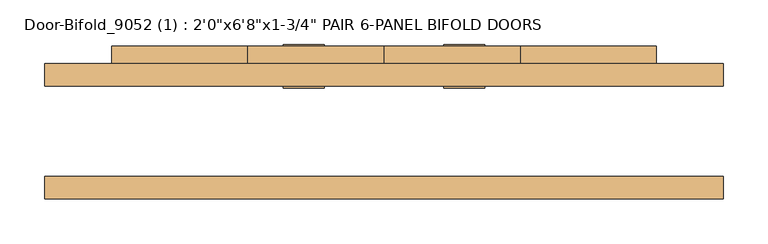
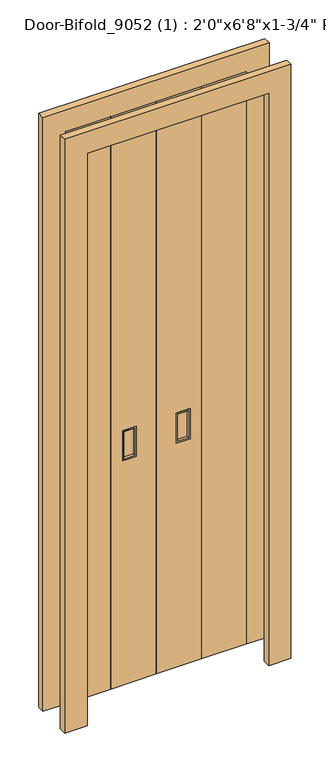
"""IFC4 building model written with IfcOpenShell, lengths in millimetres: door geometry."""

from ifc_helpers import new_model, si_unit, frame, origin, origin_with_axes, place, context, project, spatial, polyline, outline, extrude, faceted_brep, source, transform, mapped, element, save


def door_f8bdd619(model_context):
    return source(origin(), model_context, "Body", "SolidModel", [
        extrude(outline(polyline([(2032.0, -304.8), (2032.0, 304.8), (0.0, 304.8), (0.0, 379.8), (2107.0, 379.8), (2107.0, -379.8), (0.0, -379.8), (0.0, -304.8), (2032.0, -304.8)])), frame((0.0, 50.8, 0.0), z_axis=(0.0, 1.0, 0.0), x_axis=(0.0, 0.0, 1.0)), (0.0, 0.0, 1.0), 25.0),
        extrude(outline(polyline([(2107.0, -379.8), (0.0, -379.8), (0.0, -304.8), (2032.0, -304.8), (2032.0, 304.8), (0.0, 304.8), (0.0, 379.8), (2107.0, 379.8), (2107.0, -379.8)])), frame((0.0, -75.8, 0.0), z_axis=(0.0, 1.0, 0.0), x_axis=(0.0, 0.0, 1.0)), (0.0, 0.0, 1.0), 25.0),
        faceted_brep([(152.4, 50.8, 0.0), (0.0, 50.8, 0.0), (0.0, 95.25, 0.0), (152.4, 95.25, 0.0), (152.4, 50.8, 2032.0), (0.0, 50.8, 2032.0), (110.0, 50.8, 800.0), (70.0, 50.8, 800.0), (70.0, 50.8, 900.0), (110.0, 50.8, 900.0), (0.0, 95.25, 2032.0), (152.4, 95.25, 2032.0), (70.0, 95.25, 800.0), (110.0, 95.25, 800.0), (110.0, 95.25, 900.0), (70.0, 95.25, 900.0), (70.0, 85.25, 800.0), (110.0, 85.25, 800.0), (110.0, 85.25, 900.0), (70.0, 85.25, 900.0), (110.0, 60.8, 800.0), (70.0, 60.8, 800.0), (70.0, 60.8, 900.0), (110.0, 60.8, 900.0)], [[[0, 1, 2, 3]], [[4, 5, 1, 0], [6, 7, 8, 9]], [[5, 10, 2, 1]], [[10, 11, 3, 2], [12, 13, 14, 15]], [[11, 4, 0, 3]], [[16, 17, 13, 12]], [[17, 18, 14, 13]], [[18, 19, 15, 14]], [[19, 16, 12, 15]], [[20, 21, 7, 6]], [[21, 22, 8, 7]], [[22, 23, 9, 8]], [[23, 20, 6, 9]], [[16, 19, 18, 17]], [[20, 23, 22, 21]], [[4, 11, 10, 5]]]),
        faceted_brep([(0.0, 50.8, 0.0), (-152.4, 50.8, 0.0), (-152.4, 95.25, 0.0), (0.0, 95.25, 0.0), (0.0, 50.8, 2032.0), (-152.4, 50.8, 2032.0), (-70.0, 50.8, 900.0), (-70.0, 50.8, 800.0), (-110.0, 50.8, 800.0), (-110.0, 50.8, 900.0), (-152.4, 95.25, 2032.0), (0.0, 95.25, 2032.0), (-110.0, 95.25, 800.0), (-70.0, 95.25, 800.0), (-70.0, 95.25, 900.0), (-110.0, 95.25, 900.0), (-110.0, 85.25, 800.0), (-70.0, 85.25, 800.0), (-70.0, 85.25, 900.0), (-110.0, 85.25, 900.0), (-70.0, 60.8, 900.0), (-70.0, 60.8, 800.0), (-110.0, 60.8, 800.0), (-110.0, 60.8, 900.0)], [[[0, 1, 2, 3]], [[4, 5, 1, 0], [6, 7, 8, 9]], [[5, 10, 2, 1]], [[10, 11, 3, 2], [12, 13, 14, 15]], [[11, 4, 0, 3]], [[16, 17, 13, 12]], [[17, 18, 14, 13]], [[18, 19, 15, 14]], [[19, 16, 12, 15]], [[20, 21, 7, 6]], [[21, 22, 8, 7]], [[22, 23, 9, 8]], [[23, 20, 6, 9]], [[16, 19, 18, 17]], [[20, 23, 22, 21]], [[4, 11, 10, 5]]]),
        extrude(outline(polyline([(304.8, 95.25), (304.8, 50.8), (152.4, 50.8), (152.4, 95.25), (304.8, 95.25)])), origin_with_axes(), (0.0, 0.0, 1.0), 2032.0),
        extrude(outline(polyline([(-152.4, 95.25), (-152.4, 50.8), (-304.8, 50.8), (-304.8, 95.25), (-152.4, 95.25)])), origin_with_axes(), (0.0, 0.0, 1.0), 2032.0),
        extrude(outline(polyline([(108.0022505, 57.666881), (71.9977495, 57.666881), (71.9977495, 60.8), (108.0022505, 60.8), (108.0022505, 57.666881)])), frame((0.0, 0.0, 801.9977495), z_axis=(0.0, 0.0, 1.0), x_axis=(1.0, 0.0, 0.0)), (0.0, 0.0, 1.0), 96.004501),
        faceted_brep([(110.0, 60.8, 800.0), (110.0, 50.8, 800.0), (70.0, 50.8, 800.0), (70.0, 60.8, 800.0), (108.0022505, 48.8449345, 801.9977495), (108.0022505, 60.8, 801.9977495), (71.9977495, 60.8, 801.9977495), (71.9977495, 48.8449345, 801.9977495), (113.0022505, 50.8, 796.9977495), (113.0022505, 48.8449345, 796.9977495), (66.9977495, 48.8449345, 796.9977495), (66.9977495, 50.8, 796.9977495), (70.0, 50.8, 900.0), (70.0, 60.8, 900.0), (71.9977495, 60.8, 898.0022505), (71.9977495, 48.8449345, 898.0022505), (66.9977495, 48.8449345, 903.0022505), (66.9977495, 50.8, 903.0022505), (110.0, 50.8, 900.0), (110.0, 60.8, 900.0), (108.0022505, 60.8, 898.0022505), (108.0022505, 48.8449345, 898.0022505), (113.0022505, 48.8449345, 903.0022505), (113.0022505, 50.8, 903.0022505)], [[[0, 1, 2, 3]], [[4, 5, 6, 7]], [[8, 9, 10, 11]], [[3, 2, 12, 13]], [[7, 6, 14, 15]], [[11, 10, 16, 17]], [[13, 12, 18, 19]], [[15, 14, 20, 21]], [[17, 16, 22, 23]], [[11, 17, 23, 8], [1, 18, 12, 2]], [[19, 18, 1, 0]], [[3, 13, 19, 0], [5, 20, 14, 6]], [[21, 20, 5, 4]], [[9, 22, 16, 10], [7, 15, 21, 4]], [[23, 22, 9, 8]]]),
        extrude(outline(polyline([(-108.0022505, 60.8), (-71.9977495, 60.8), (-71.9977495, 57.666881), (-108.0022505, 57.666881), (-108.0022505, 60.8)])), frame((0.0, 0.0, 801.9977495), z_axis=(0.0, 0.0, 1.0), x_axis=(1.0, 0.0, 0.0)), (0.0, 0.0, 1.0), 96.004501),
        faceted_brep([(-70.0, 60.8, 800.0), (-70.0, 50.8, 800.0), (-110.0, 50.8, 800.0), (-110.0, 60.8, 800.0), (-71.9977495, 48.8449345, 801.9977495), (-71.9977495, 60.8, 801.9977495), (-108.0022505, 60.8, 801.9977495), (-108.0022505, 48.8449345, 801.9977495), (-66.9977495, 50.8, 796.9977495), (-66.9977495, 48.8449345, 796.9977495), (-113.0022505, 48.8449345, 796.9977495), (-113.0022505, 50.8, 796.9977495), (-110.0, 50.8, 900.0), (-110.0, 60.8, 900.0), (-108.0022505, 60.8, 898.0022505), (-108.0022505, 48.8449345, 898.0022505), (-113.0022505, 48.8449345, 903.0022505), (-113.0022505, 50.8, 903.0022505), (-70.0, 50.8, 900.0), (-70.0, 60.8, 900.0), (-71.9977495, 60.8, 898.0022505), (-71.9977495, 48.8449345, 898.0022505), (-66.9977495, 48.8449345, 903.0022505), (-66.9977495, 50.8, 903.0022505)], [[[0, 1, 2, 3]], [[4, 5, 6, 7]], [[8, 9, 10, 11]], [[3, 2, 12, 13]], [[7, 6, 14, 15]], [[11, 10, 16, 17]], [[13, 12, 18, 19]], [[15, 14, 20, 21]], [[17, 16, 22, 23]], [[11, 17, 23, 8], [1, 18, 12, 2]], [[19, 18, 1, 0]], [[3, 13, 19, 0], [5, 20, 14, 6]], [[21, 20, 5, 4]], [[9, 22, 16, 10], [7, 15, 21, 4]], [[23, 22, 9, 8]]]),
        extrude(outline(polyline([(-71.9977495, 85.25), (-108.0022505, 85.25), (-108.0022505, 88.5598365), (-71.9977495, 88.5598365), (-71.9977495, 85.25)])), frame((0.0, 0.0, 801.9977495), z_axis=(0.0, 0.0, 1.0), x_axis=(1.0, 0.0, 0.0)), (0.0, 0.0, 1.0), 96.004501),
        extrude(outline(polyline([(108.0022505, 85.25), (71.9977495, 85.25), (71.9977495, 88.5598365), (108.0022505, 88.5598365), (108.0022505, 85.25)])), frame((0.0, 0.0, 801.9977495), z_axis=(0.0, 0.0, 1.0), x_axis=(1.0, 0.0, 0.0)), (0.0, 0.0, 1.0), 96.004501),
        faceted_brep([(110.0, 85.25, 900.0), (110.0, 95.25, 900.0), (70.0, 95.25, 900.0), (70.0, 85.25, 900.0), (108.0022505, 97.2050655, 898.0022505), (108.0022505, 85.25, 898.0022505), (71.9977495, 85.25, 898.0022505), (71.9977495, 97.2050655, 898.0022505), (113.0022505, 95.25, 903.0022505), (113.0022505, 97.2050655, 903.0022505), (66.9977495, 97.2050655, 903.0022505), (66.9977495, 95.25, 903.0022505), (70.0, 95.25, 800.0), (70.0, 85.25, 800.0), (71.9977495, 85.25, 801.9977495), (71.9977495, 97.2050655, 801.9977495), (66.9977495, 97.2050655, 796.9977495), (66.9977495, 95.25, 796.9977495), (110.0, 95.25, 800.0), (110.0, 85.25, 800.0), (108.0022505, 85.25, 801.9977495), (108.0022505, 97.2050655, 801.9977495), (113.0022505, 97.2050655, 796.9977495), (113.0022505, 95.25, 796.9977495)], [[[0, 1, 2, 3]], [[4, 5, 6, 7]], [[8, 9, 10, 11]], [[3, 2, 12, 13]], [[7, 6, 14, 15]], [[11, 10, 16, 17]], [[13, 12, 18, 19]], [[15, 14, 20, 21]], [[17, 16, 22, 23]], [[11, 17, 23, 8], [1, 18, 12, 2]], [[19, 18, 1, 0]], [[3, 13, 19, 0], [5, 20, 14, 6]], [[21, 20, 5, 4]], [[9, 22, 16, 10], [7, 15, 21, 4]], [[23, 22, 9, 8]]]),
        faceted_brep([(-70.0, 85.25, 900.0), (-70.0, 95.25, 900.0), (-110.0, 95.25, 900.0), (-110.0, 85.25, 900.0), (-71.9977495, 97.2050655, 898.0022505), (-71.9977495, 85.25, 898.0022505), (-108.0022505, 85.25, 898.0022505), (-108.0022505, 97.2050655, 898.0022505), (-66.9977495, 95.25, 903.0022505), (-66.9977495, 97.2050655, 903.0022505), (-113.0022505, 97.2050655, 903.0022505), (-113.0022505, 95.25, 903.0022505), (-110.0, 95.25, 800.0), (-110.0, 85.25, 800.0), (-108.0022505, 85.25, 801.9977495), (-108.0022505, 97.2050655, 801.9977495), (-113.0022505, 97.2050655, 796.9977495), (-113.0022505, 95.25, 796.9977495), (-70.0, 95.25, 800.0), (-70.0, 85.25, 800.0), (-71.9977495, 85.25, 801.9977495), (-71.9977495, 97.2050655, 801.9977495), (-66.9977495, 97.2050655, 796.9977495), (-66.9977495, 95.25, 796.9977495)], [[[0, 1, 2, 3]], [[4, 5, 6, 7]], [[8, 9, 10, 11]], [[3, 2, 12, 13]], [[7, 6, 14, 15]], [[11, 10, 16, 17]], [[13, 12, 18, 19]], [[15, 14, 20, 21]], [[17, 16, 22, 23]], [[11, 17, 23, 8], [1, 18, 12, 2]], [[19, 18, 1, 0]], [[3, 13, 19, 0], [5, 20, 14, 6]], [[21, 20, 5, 4]], [[9, 22, 16, 10], [7, 15, 21, 4]], [[23, 22, 9, 8]]]),
    ])


if __name__ == "__main__":
    model = new_model("IFC4")
    model_context = context("Model", 3, world=origin())
    ifc_project = project(units=[si_unit("LENGTHUNIT", "METRE", prefix="MILLI")], contexts=[model_context])
    site = spatial("IfcSite", under=ifc_project)
    building = spatial("IfcBuilding", under=site)
    placement = place(None, origin())
    door_shape = door_f8bdd619(model_context)
    element("IfcDoor", 1, ObjectType="Door-Bifold_9052 (1) : 2'0\"x6'8\"x1-3/4\" PAIR 6-PANEL BIFOLD DOORS", at=placement, inside=building, context=model_context, shape_type="MappedRepresentation", body=[
        mapped(door_shape, transform((0.0, 0.0, 0.0), x_axis=(1.0, 0.0, 0.0), y_axis=(0.0, 1.0, 0.0), z_axis=(0.0, 0.0, 1.0))),
    ])
    save(model, "model.ifc")

# Revit data of these elements
# Type "Door-Bifold_9052 (1) : 2'0\"x6'8\"x1-3/4\" PAIR 6-PANEL BIFOLD DOORS"
#   Type Mark = "25"
#   Model = "Porta de Fole"
#   Manufacturer = "Typhoon"
#   Thickness = 0' - 1 3/4"
#   Frame Projection Ext. = 0' - 0.98425"
#   Frame Projection Int. = 0' - 0.98425"
#   Frame Width = 0' - 2.95276"
#   Height = 6' - 8"
#   Width = 2' - 0"
#   Comp_painel = 0' - 6"
#   Abertura = 0.00°
#   Altura Puxador = 2' - 11.43307"
#   Puxador = Puxador
#   Painel-Porta = Porta-Painel
#   Function = (empty or 0)
#   Wall Closure = (empty or 0)
# Element 1 (IfcDoor, "Door-Bifold_9052 (1) : 2'0\"x6'8\"x1-3/4\" PAIR 6-PANEL BIFOLD DOORS")
#   Materials on its faces: "Puxador", "Porta-Painel"
# Materials
#   "Puxador": class "Metal", colour RGB 244 244 244, transparency 0
#   "Porta-Painel": class "Wood", colour RGB 135 74 45, transparency 0
